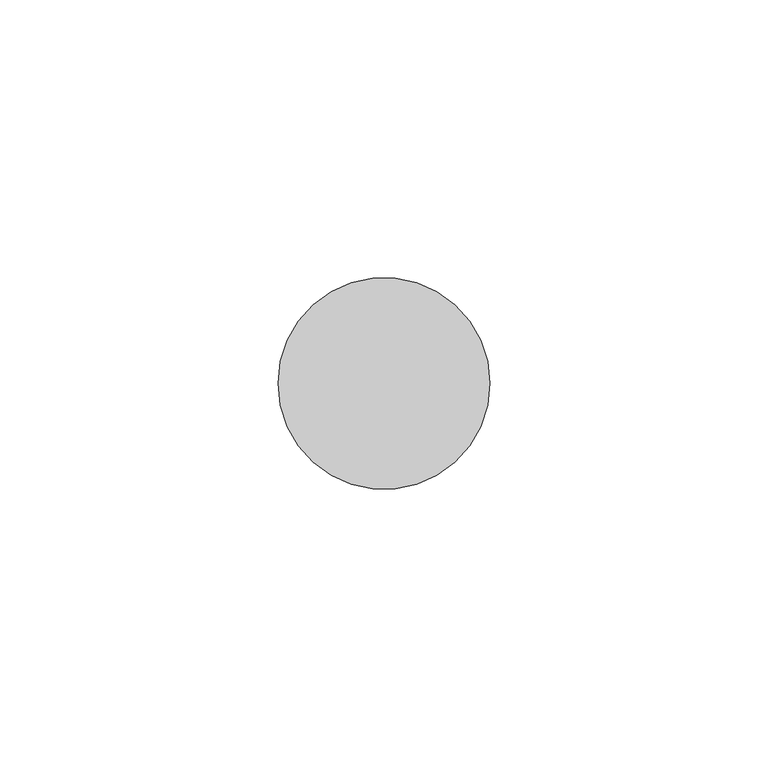
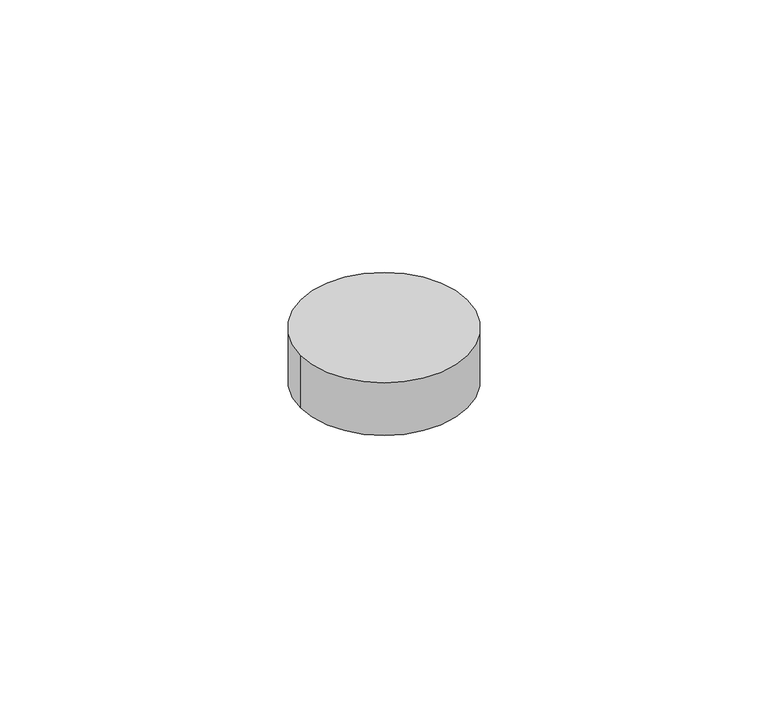
"""IFC4 building model written with IfcOpenShell, lengths in millimetres: proxy geometry, Bolt4:Bolt001:302941 : Bolt4:Bolt001:302941."""

from ifc_helpers import new_model, si_unit, point, frame, frame_2d, origin, place, context, project, spatial, circle_curve, trimmed, segment, composite_curve, outline, extrude, source, transform, mapped, element, save


def generic_models_a4505f7c(model_context):
    return source(origin(), model_context, "Body", "SweptSolid", [
        extrude(outline(composite_curve([segment(trimmed(circle_curve(frame_2d((12028.9793228, -1503.5124296)), 19.05), [point((12009.9293228, -1503.5124296))], [point((12048.0293228, -1503.5124296))], False, "CARTESIAN"), True, "CONTINUOUS"), segment(trimmed(circle_curve(frame_2d((12028.9793228, -1503.5124296)), 19.05), [point((12048.0293228, -1503.5124296))], [point((12009.9293228, -1503.5124296))], False, "CARTESIAN"), True, "CONTINUOUS")], self_intersect=False)), frame((0.0, 0.0, 40068.246), z_axis=(0.0, 0.0, 1.0), x_axis=(1.0, 0.0, 0.0)), (0.0, 0.0, 1.0), 12.7),
    ])


if __name__ == "__main__":
    model = new_model("IFC4")
    model_context = context("Model", 3, world=origin())
    ifc_project = project(units=[si_unit("LENGTHUNIT", "METRE", prefix="MILLI")], contexts=[model_context])
    site = spatial("IfcSite", under=ifc_project)
    building = spatial("IfcBuilding", under=site)
    placement = place(None, origin())
    generic_models_shape = generic_models_a4505f7c(model_context)
    element("IfcBuildingElementProxy", 1, Name="Bolt4:Bolt001:302941 : Bolt4:Bolt001:302941", ObjectType="Bolt4:Bolt001:302941 : Bolt4:Bolt001:302941", at=placement, inside=building, context=model_context, shape_type="MappedRepresentation", body=[
        mapped(generic_models_shape, transform((0.0, 0.0, 0.0), x_axis=(1.0, 0.0, 0.0), y_axis=(0.0, 1.0, 0.0), z_axis=(0.0, 0.0, 1.0))),
    ])
    save(model, "model.ifc")

# Revit data of these elements
# Type "Bolt4:Bolt001:302941 : Bolt4:Bolt001:302941"
#   NameOverride = "Bolt4:Bolt001:302941"
#   ObjectTypeOverride = "Bolt4:Bolt001"
#   Reference = "Bolt001"
#   Category = "Generic Models"
#   Tag = "302941"
# Element 1 (IfcBuildingElementProxy, "Bolt4:Bolt001:302941 : Bolt4:Bolt001:302941")
#   Materials on its faces: "BOLTS CONCEALED BY FLOOR FINISH"
# Materials
#   "BOLTS CONCEALED BY FLOOR FINISH": class "Unassigned", colour RGB 128 128 128, transparency 0
